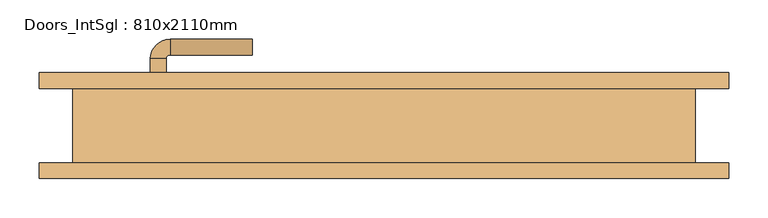
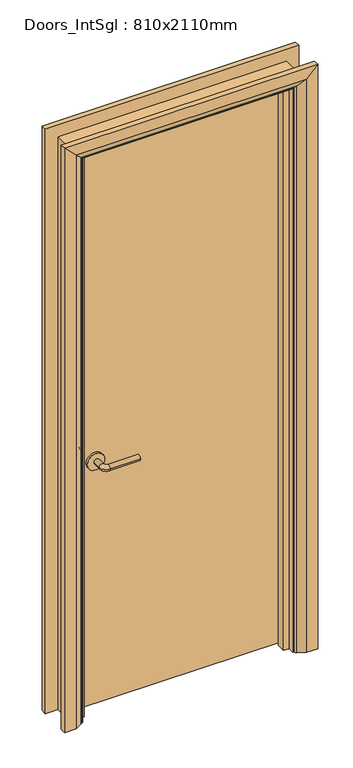
"""IFC4 building model written with IfcOpenShell, lengths in millimetres: door geometry, Doors_IntSgl : 810x2110mm."""

import ifcopenshell
import ifcopenshell.guid

model = None  # the IFC model being written
_history = None  # IfcOwnerHistory: only IFC2X3 demands one
_inside = {}  # id of a spatial element -> (the spatial element, [elements in it])
_under = {}  # id of a project, library or spatial element -> (it, [spatial elements below it])
_declared = {}  # id of a project -> (the project, [libraries it declares])
_typed = {}  # id of a type object -> (the type object, [elements of that type])
_made_of = {}  # id of a material, layer set ... -> (it, [elements and type objects made of it])


def new_model(schema):
    """Start an empty IFC model of exactly this schema.

    Asked for "IFC4X3", IfcOpenShell would pick the latest addendum, in which some entities
    have other attributes; the version numbers below select the first issue.
    IFC2X3 requires an IfcOwnerHistory on every rooted entity: one is made here for all.
    """
    global model, _history
    if schema == "IFC4X3":
        model = ifcopenshell.file(schema_version=(4, 3, 0, 0))
    else:
        model = ifcopenshell.file(schema=schema)
    _inside.clear()
    _under.clear()
    _declared.clear()
    _typed.clear()
    _made_of.clear()
    _history = None
    if model.schema == "IFC2X3":
        org = make("IfcOrganization", Name="unknown")
        user = make(
            "IfcPersonAndOrganization",
            ThePerson=make("IfcPerson", FamilyName="unknown"),
            TheOrganization=org,
        )
        app = make(
            "IfcApplication",
            ApplicationDeveloper=org,
            Version="unknown",
            ApplicationFullName="unknown",
            ApplicationIdentifier="unknown",
        )
        _history = make(
            "IfcOwnerHistory",
            OwningUser=user,
            OwningApplication=app,
            ChangeAction="ADDED",
            CreationDate=0,
        )
    return model


def make(cls, **values):
    """One entity of the class cls with the attributes given. An attribute that is None is left unset."""
    return model.create_entity(
        cls, **{name: value for name, value in values.items() if value is not None}
    )


def rooted(cls, **values):
    """An entity with a GlobalId (a new one), such as an element, a storey or a relation."""
    return make(cls, GlobalId=ifcopenshell.guid.new(), OwnerHistory=_history, **values)


def si_unit(unit_type, name, prefix=None):
    """IfcSIUnit, for example si_unit("LENGTHUNIT", "METRE", prefix="MILLI")."""
    return make("IfcSIUnit", UnitType=unit_type, Prefix=prefix, Name=name)


def assignment(units):
    """IfcUnitAssignment: the units of a project."""
    return None if units is None else make("IfcUnitAssignment", Units=units)


def point(xyz):
    """IfcCartesianPoint."""
    return None if xyz is None else make("IfcCartesianPoint", Coordinates=xyz)


def direction(xyz):
    """IfcDirection."""
    return None if xyz is None else make("IfcDirection", DirectionRatios=xyz)


def frame(location, z_axis=None, x_axis=None):
    """IfcAxis2Placement3D, a coordinate frame: its origin and axes. An axis left out is left unset."""
    return make(
        "IfcAxis2Placement3D",
        Location=point(location),
        Axis=direction(z_axis),
        RefDirection=direction(x_axis),
    )


def frame_2d(location, x_axis=None):
    """IfcAxis2Placement2D, a coordinate frame in the plane: its origin and x axis."""
    return make(
        "IfcAxis2Placement2D", Location=point(location), RefDirection=direction(x_axis)
    )


def origin():
    """The frame at (0, 0, 0) with its axes left unset."""
    return frame((0.0, 0.0, 0.0))


def place(relative_to, where):
    """IfcLocalPlacement: puts the frame where relative to a parent placement (None: the world)."""
    return make(
        "IfcLocalPlacement", PlacementRelTo=relative_to, RelativePlacement=where
    )


def context(
    kind, dimensions, precision=None, world=None, true_north=None, identifier=None
):
    """IfcGeometricRepresentationContext, for example the 3D "Model" context."""
    return make(
        "IfcGeometricRepresentationContext",
        ContextIdentifier=identifier,
        ContextType=kind,
        CoordinateSpaceDimension=dimensions,
        Precision=precision,
        WorldCoordinateSystem=world,
        TrueNorth=true_north,
    )


def project(units=None, contexts=None):
    """IfcProject with its units and contexts."""
    return rooted(
        "IfcProject",
        Name="project",
        RepresentationContexts=contexts,
        UnitsInContext=assignment(units),
    )


def spatial(cls, under=None, at=None, **own):
    """A site, building, storey or space (cls), placed at a placement, below another one or the project."""
    s = rooted(cls, ObjectPlacement=at, **own)
    if under is not None:
        _under.setdefault(under.id(), (under, []))[1].append(s)
    return s


def polyline(points):
    """IfcPolyline through the points."""
    return make("IfcPolyline", Points=[point(p) for p in points])


def circle_curve(where, radius):
    """IfcCircle in the frame where."""
    return make("IfcCircle", Position=where, Radius=radius)


def ellipse_curve(where, semi_axis1, semi_axis2):
    """IfcEllipse in the frame where."""
    return make(
        "IfcEllipse", Position=where, SemiAxis1=semi_axis1, SemiAxis2=semi_axis2
    )


def trimmed(basis, trim1, trim2, sense, master):
    """IfcTrimmedCurve: the piece of a basis curve between two trims."""
    return make(
        "IfcTrimmedCurve",
        BasisCurve=basis,
        Trim1=trim1,
        Trim2=trim2,
        SenseAgreement=sense,
        MasterRepresentation=master,
    )


def segment(curve, same_sense, transition):
    """IfcCompositeCurveSegment."""
    return make(
        "IfcCompositeCurveSegment",
        Transition=transition,
        SameSense=same_sense,
        ParentCurve=curve,
    )


def composite_curve(segments, self_intersect=None):
    """IfcCompositeCurve: segments joined end to end."""
    return make("IfcCompositeCurve", Segments=segments, SelfIntersect=self_intersect)


def outline(outer, holes=None, kind="AREA"):
    """IfcArbitraryClosedProfileDef: a profile drawn as a closed curve; with holes, ...WithVoids."""
    if holes is None:
        return make("IfcArbitraryClosedProfileDef", ProfileType=kind, OuterCurve=outer)
    return make(
        "IfcArbitraryProfileDefWithVoids",
        ProfileType=kind,
        OuterCurve=outer,
        InnerCurves=holes,
    )


def extrude(swept, where, along, depth):
    """IfcExtrudedAreaSolid: the profile swept, set in the frame where, extruded along a direction by depth."""
    return make(
        "IfcExtrudedAreaSolid",
        SweptArea=swept,
        Position=where,
        ExtrudedDirection=direction(along),
        Depth=depth,
    )


def faces_of(points, faces, orient=None, outer=None):
    """IfcFace entities. A face is a list of loops; a loop is a list of indices into points, from 0.

    orient and outer hold one flag for each loop. By default every Orientation is true, the
    first loop of a face is its IfcFaceOuterBound and the others are IfcFaceBound.
    """
    made = []
    for i, loops in enumerate(faces):
        bounds = []
        for j, loop in enumerate(loops):
            is_outer = j == 0 if outer is None else outer[i][j]
            bounds.append(
                make(
                    "IfcFaceOuterBound" if is_outer else "IfcFaceBound",
                    Bound=make("IfcPolyLoop", Polygon=[points[k] for k in loop]),
                    Orientation=True if orient is None else orient[i][j],
                )
            )
        made.append(make("IfcFace", Bounds=bounds))
    return made


def faceted_brep(points, faces, orient=None, outer=None, voids=None):
    """IfcFacetedBrep: a solid bounded by flat faces; with voids (closed shells), ...WithVoids."""
    shared = [point(p) for p in points]
    hull = make("IfcClosedShell", CfsFaces=faces_of(shared, faces, orient, outer))
    if voids is None:
        return make("IfcFacetedBrep", Outer=hull)
    return make(
        "IfcFacetedBrepWithVoids",
        Outer=hull,
        Voids=[
            make(cls, CfsFaces=faces_of(shared, fs, o, b)) for cls, fs, o, b in voids
        ],
    )


def shape(context_of_items, identifier, shape_type, items):
    """IfcShapeRepresentation: the items that make up one representation, for example the "Body"."""
    return make(
        "IfcShapeRepresentation",
        ContextOfItems=context_of_items,
        RepresentationIdentifier=identifier,
        RepresentationType=shape_type,
        Items=items,
    )


def source(mapping_origin, context_of_items, identifier, shape_type, items):
    """IfcRepresentationMap: a shape defined once, which mapped items show again and again."""
    return make(
        "IfcRepresentationMap",
        MappingOrigin=mapping_origin,
        MappedRepresentation=shape(context_of_items, identifier, shape_type, items),
    )


def transform(
    local_origin,
    x_axis=None,
    y_axis=None,
    z_axis=None,
    scale=None,
    scale2=None,
    scale3=None,
    uniform=True,
):
    """IfcCartesianTransformationOperator3D, or its non-uniform kind. x_axis, y_axis, z_axis: its Axis1, 2, 3."""
    if uniform:
        return make(
            "IfcCartesianTransformationOperator3D",
            Axis1=direction(x_axis),
            Axis2=direction(y_axis),
            LocalOrigin=point(local_origin),
            Scale=scale,
            Axis3=direction(z_axis),
        )
    return make(
        "IfcCartesianTransformationOperator3DnonUniform",
        Axis1=direction(x_axis),
        Axis2=direction(y_axis),
        LocalOrigin=point(local_origin),
        Scale=scale,
        Axis3=direction(z_axis),
        Scale2=scale2,
        Scale3=scale3,
    )


def mapped(mapping_source, mapping_target):
    """IfcMappedItem: shows the shape of a source again, moved by a transform."""
    return make(
        "IfcMappedItem", MappingSource=mapping_source, MappingTarget=mapping_target
    )


def made_of(thing, what):
    """Note that an element or type object is made of a material, layer set ...; save() writes the relation."""
    if what is not None:
        _made_of.setdefault(what.id(), (what, []))[1].append(thing)
    return thing


def element(
    cls,
    number,
    at=None,
    inside=None,
    cuts=None,
    type_object=None,
    material=None,
    context=None,
    identifier="Body",
    shape_type=None,
    held_by="IfcProductDefinitionShape",
    body=None,
    shapes=None,
    **own,
):
    """One element of the class cls, such as IfcWall. Its Tag is "e" and its number.

    at: its placement. inside: the storey or other place that contains it. cuts: it is an
    opening in that element (IfcRelVoidsElement). A single representation is given by context,
    identifier, shape_type and body (its items); several are given by shapes. held_by: the class
    of the entity that holds the representations. save() writes the other relations.
    """
    e = rooted(cls, Tag="e%d" % number, ObjectPlacement=at, **own)
    if body is not None:
        shapes = [shape(context, identifier, shape_type, body)]
    if shapes is not None:
        e.Representation = make(held_by, Representations=shapes)
    if inside is not None:
        _inside.setdefault(inside.id(), (inside, []))[1].append(e)
    if cuts is not None:
        rooted(
            "IfcRelVoidsElement", RelatingBuildingElement=cuts, RelatedOpeningElement=e
        )
    if type_object is not None:
        _typed.setdefault(type_object.id(), (type_object, []))[1].append(e)
    return made_of(e, material)


def aggregate(whole, parts):
    """IfcRelAggregates: a whole, such as a stair, and the parts it consists of."""
    return rooted("IfcRelAggregates", RelatingObject=whole, RelatedObjects=parts)


def save(model, path):
    """Write the relations noted so far, then the file.

    IfcRelAggregates (storeys below a building ...), IfcRelContainedInSpatialStructure (elements
    in a storey), IfcRelDefinesByType, IfcRelAssociatesMaterial and IfcRelDeclares: one each for
    every whole, place, type object, material and project.
    """
    for whole, parts in _under.values():
        aggregate(whole, parts)
    for where, things in _inside.values():
        rooted(
            "IfcRelContainedInSpatialStructure",
            RelatedElements=things,
            RelatingStructure=where,
        )
    for kind, things in _typed.values():
        rooted("IfcRelDefinesByType", RelatedObjects=things, RelatingType=kind)
    for what, things in _made_of.values():
        rooted("IfcRelAssociatesMaterial", RelatedObjects=things, RelatingMaterial=what)
    for by, libraries in _declared.values():
        rooted("IfcRelDeclares", RelatingContext=by, RelatedDefinitions=libraries)
    model.write(path)


def plane_surface(at):
    """IfcPlane: the flat surface through the origin of the frame at, square to its z axis."""
    return make("IfcPlane", Position=at)


def cylinder_surface(at, radius):
    """IfcCylindricalSurface: all points at the distance radius from the z axis of the frame at."""
    return make("IfcCylindricalSurface", Position=at, Radius=radius)


def revolved_surface(curve, axis_point, axis_direction):
    """IfcSurfaceOfRevolution: the curve turned about the line through axis_point along axis_direction."""
    return make(
        "IfcSurfaceOfRevolution",
        SweptCurve=make("IfcArbitraryOpenProfileDef", ProfileType="CURVE", Curve=curve),
        AxisPosition=make("IfcAxis1Placement", Location=point(axis_point), Axis=direction(axis_direction)),
    )


def advanced_brep(points, edges, surfaces, faces):
    """IfcAdvancedBrep: a solid bounded by faces that lie on surfaces and meet in shared edges.

    An edge is (start, end): straight between two places in points (the first is 0);
    or (start, end, curve); or (start, end, curve, False) where it runs against its curve.
    A face is (place in surfaces, loops), or (place, loops, False) where it looks against
    its surface's normal. A loop lists edges by number (the first is 1), with a minus sign
    where the edge is run from its end to its start. The first loop is the outer one.
    """
    corners = [point(p) for p in points]
    vertices = [make("IfcVertexPoint", VertexGeometry=c) for c in corners]
    made = []
    for start, end, *more in edges:
        made.append(
            make(
                "IfcEdgeCurve",
                EdgeStart=vertices[start],
                EdgeEnd=vertices[end],
                EdgeGeometry=more[0] if more else make("IfcPolyline", Points=[corners[start], corners[end]]),
                SameSense=more[1] if len(more) > 1 else True,
            )
        )
    hull = []
    for where, loops, *sense in faces:
        bounds = []
        for j, loop in enumerate(loops):
            ring = [make("IfcOrientedEdge", EdgeElement=made[abs(k) - 1], Orientation=k > 0) for k in loop]
            bounds.append(
                make(
                    "IfcFaceOuterBound" if j == 0 else "IfcFaceBound",
                    Bound=make("IfcEdgeLoop", EdgeList=ring),
                    Orientation=True,
                )
            )
        hull.append(make("IfcAdvancedFace", Bounds=bounds, FaceSurface=surfaces[where], SameSense=sense[0] if sense else True))
    return make("IfcAdvancedBrep", Outer=make("IfcClosedShell", CfsFaces=hull))


def doors_intsgl_810x2110mm_acea5367(model_context):
    return source(origin(), model_context, "Body", "SolidModel", [
        advanced_brep(
        [(-298.0, 1.5, 900.0), (-278.0, 1.5, 900.0), (-278.0, -28.5, 900.0), (-298.0, -28.5, 900.0), (-273.0, -33.5, 900.0), (-273.0, -53.5, 900.0), (-168.0, -53.5, 900.0), (-168.0, -33.5, 900.0)],
        [
            (0, 1, circle_curve(frame((-288.0, 1.5, 900.0), z_axis=(0.0, 1.0, 0.0), x_axis=(1.0, 0.0, 0.0)), 10.0)),
            (1, 0, circle_curve(frame((-288.0, 1.5, 900.0), z_axis=(0.0, 1.0, 0.0), x_axis=(1.0, 0.0, 0.0)), 10.0)),
            (1, 2),
            (2, 3, circle_curve(frame((-288.0, -28.5, 900.0), z_axis=(0.0, 1.0, 0.0), x_axis=(1.0, 0.0, 0.0)), 10.0)),
            (3, 0),
            (3, 2, circle_curve(frame((-288.0, -28.5, 900.0), z_axis=(0.0, 1.0, 0.0), x_axis=(1.0, 0.0, 0.0)), 10.0)),
            (4, 5, circle_curve(frame((-273.0, -43.5, 900.0), z_axis=(-1.0, 0.0, 0.0), x_axis=(0.0, 1.0, 0.0)), 10.0)),
            (5, 3, circle_curve(frame((-273.0, -28.5, 900.0), z_axis=(0.0, 0.0, -1.0), x_axis=(-1.0, 0.0, 0.0)), 25.0)),
            (2, 4, circle_curve(frame((-273.0, -28.5, 900.0), z_axis=(0.0, 0.0, 1.0), x_axis=(-1.0, 0.0, 0.0)), 5.0)),
            (5, 4, circle_curve(frame((-273.0, -43.5, 900.0), z_axis=(-1.0, 0.0, 0.0), x_axis=(0.0, 1.0, 0.0)), 10.0)),
            (6, 7, circle_curve(frame((-168.0, -43.5, 900.0), z_axis=(1.0, 0.0, 0.0), x_axis=(0.0, 1.0, 0.0)), 10.0)),
            (7, 6, circle_curve(frame((-168.0, -43.5, 900.0), z_axis=(1.0, 0.0, 0.0), x_axis=(0.0, 1.0, 0.0)), 10.0)),
            (4, 7),
            (6, 5),
        ],
        [
            plane_surface(frame((-288.0, 1.5, 900.0), z_axis=(0.0, 1.0, 0.0), x_axis=(0.0, 0.0, 1.0))),
            cylinder_surface(frame((-288.0, 1.5, 900.0), z_axis=(0.0, 1.0, 0.0), x_axis=(1.0, 0.0, 0.0)), 10.0),
            revolved_surface(trimmed(ellipse_curve(frame((-288.0, -28.5, 900.0), z_axis=(0.0, -1.0, 0.0), x_axis=(1.0, 0.0, 0.0)), 10.0, 10.0), [point((-298.0, -28.5, 900.0))], [point((-278.0, -28.5, 900.0))], True, "CARTESIAN"), (-273.0, -28.5, 900.0), (0.0, 0.0, -1.0)),
            revolved_surface(trimmed(ellipse_curve(frame((-288.0, -28.5, 900.0), z_axis=(0.0, -1.0, 0.0), x_axis=(1.0, 0.0, 0.0)), 10.0, 10.0), [point((-278.0, -28.5, 900.0))], [point((-298.0, -28.5, 900.0))], True, "CARTESIAN"), (-273.0, -28.5, 900.0), (0.0, 0.0, -1.0)),
            plane_surface(frame((-168.0, -43.5, 900.0), z_axis=(1.0, 0.0, 0.0), x_axis=(0.0, 0.0, 1.0))),
            cylinder_surface(frame((-273.0, -43.5, 900.0), z_axis=(-1.0, 0.0, 0.0), x_axis=(0.0, 1.0, 0.0)), 10.0),
        ],
        [
            (0, [[1, 2]]),
            (1, [[3, 4, 5, -2]]),
            (1, [[-5, 6, -3, -1]]),
            (2, [[7, 8, -4, 9]]),
            (3, [[10, -9, -6, -8]]),
            (4, [[11, 12]]),
            (5, [[13, -11, 14, -7]]),
            (5, [[-14, -12, -13, -10]]),
        ],
    ),
        extrude(outline(composite_curve([segment(trimmed(circle_curve(frame_2d((900.0, -290.5)), 30.0), [point((900.0, -320.5))], [point((900.0, -260.5))], False, "CARTESIAN"), True, "CONTINUOUS"), segment(trimmed(circle_curve(frame_2d((900.0, -290.5)), 30.0), [point((900.0, -260.5))], [point((900.0, -320.5))], False, "CARTESIAN"), True, "CONTINUOUS")], self_intersect=False)), frame((0.0, 1.5, 0.0), z_axis=(0.0, 1.0, 0.0), x_axis=(0.0, 0.0, 1.0)), (0.0, 0.0, 1.0), 8.0),
        advanced_brep(
        [(-298.0, 55.5, 900.0), (-278.0, 55.5, 900.0), (-298.0, 85.5, 900.0), (-278.0, 85.5, 900.0), (-273.0, 90.5, 900.0), (-273.0, 110.5, 900.0), (-168.0, 110.5, 900.0), (-168.0, 90.5, 900.0)],
        [
            (0, 1, circle_curve(frame((-288.0, 55.5, 900.0), z_axis=(0.0, -1.0, 0.0), x_axis=(1.0, 0.0, 0.0)), 10.0)),
            (1, 0, circle_curve(frame((-288.0, 55.5, 900.0), z_axis=(0.0, -1.0, 0.0), x_axis=(1.0, 0.0, 0.0)), 10.0)),
            (0, 2),
            (2, 3, circle_curve(frame((-288.0, 85.5, 900.0), z_axis=(0.0, -1.0, 0.0), x_axis=(1.0, 0.0, 0.0)), 10.0)),
            (3, 1),
            (3, 2, circle_curve(frame((-288.0, 85.5, 900.0), z_axis=(0.0, -1.0, 0.0), x_axis=(1.0, 0.0, 0.0)), 10.0)),
            (4, 3, circle_curve(frame((-273.0, 85.5, 900.0), z_axis=(0.0, 0.0, 1.0), x_axis=(-1.0, 0.0, 0.0)), 5.0)),
            (2, 5, circle_curve(frame((-273.0, 85.5, 900.0), z_axis=(0.0, 0.0, -1.0), x_axis=(-1.0, 0.0, 0.0)), 25.0)),
            (5, 4, circle_curve(frame((-273.0, 100.5, 900.0), z_axis=(-1.0, 0.0, 0.0), x_axis=(0.0, -1.0, 0.0)), 10.0)),
            (4, 5, circle_curve(frame((-273.0, 100.5, 900.0), z_axis=(-1.0, 0.0, 0.0), x_axis=(0.0, -1.0, 0.0)), 10.0)),
            (6, 7, circle_curve(frame((-168.0, 100.5, 900.0), z_axis=(1.0, 0.0, 0.0), x_axis=(0.0, -1.0, 0.0)), 10.0)),
            (7, 6, circle_curve(frame((-168.0, 100.5, 900.0), z_axis=(1.0, 0.0, 0.0), x_axis=(0.0, -1.0, 0.0)), 10.0)),
            (5, 6),
            (7, 4),
        ],
        [
            plane_surface(frame((-288.0, 55.5, 900.0), z_axis=(0.0, -1.0, 0.0), x_axis=(0.0, 0.0, 1.0))),
            cylinder_surface(frame((-288.0, 55.5, 900.0), z_axis=(0.0, -1.0, 0.0), x_axis=(1.0, 0.0, 0.0)), 10.0),
            revolved_surface(trimmed(ellipse_curve(frame((-288.0, 85.5, 900.0), z_axis=(0.0, -1.0, 0.0), x_axis=(1.0, 0.0, 0.0)), 10.0, 10.0), [point((-298.0, 85.5, 900.0))], [point((-278.0, 85.5, 900.0))], True, "CARTESIAN"), (-273.0, 85.5, 900.0), (0.0, 0.0, -1.0)),
            revolved_surface(trimmed(ellipse_curve(frame((-288.0, 85.5, 900.0), z_axis=(0.0, -1.0, 0.0), x_axis=(1.0, 0.0, 0.0)), 10.0, 10.0), [point((-278.0, 85.5, 900.0))], [point((-298.0, 85.5, 900.0))], True, "CARTESIAN"), (-273.0, 85.5, 900.0), (0.0, 0.0, -1.0)),
            plane_surface(frame((-168.0, 100.5, 900.0), z_axis=(1.0, 0.0, 0.0), x_axis=(0.0, 0.0, 1.0))),
            cylinder_surface(frame((-273.0, 100.5, 900.0), z_axis=(-1.0, 0.0, 0.0), x_axis=(0.0, -1.0, 0.0)), 10.0),
        ],
        [
            (0, [[1, 2]]),
            (1, [[-1, 3, 4, 5]]),
            (1, [[-2, -5, 6, -3]]),
            (2, [[7, -4, 8, 9]]),
            (3, [[-8, -6, -7, 10]]),
            (4, [[11, 12]]),
            (5, [[-9, 13, -12, 14]]),
            (5, [[-10, -14, -11, -13]]),
        ],
    ),
        extrude(outline(composite_curve([segment(trimmed(circle_curve(frame_2d((900.0, -290.5)), 30.0), [point((900.0, -320.5))], [point((900.0, -260.5))], False, "CARTESIAN"), True, "CONTINUOUS"), segment(trimmed(circle_curve(frame_2d((900.0, -290.5)), 30.0), [point((900.0, -260.5))], [point((900.0, -320.5))], False, "CARTESIAN"), True, "CONTINUOUS")], self_intersect=False)), frame((0.0, 47.5, 0.0), z_axis=(0.0, 1.0, 0.0), x_axis=(0.0, 0.0, 1.0)), (0.0, 0.0, 1.0), 8.0),
        extrude(outline(polyline([(363.0, 9.5), (-363.0, 9.5), (-363.0, 47.5), (363.0, 47.5), (363.0, 9.5)])), frame((0.0, 0.0, 8.0), z_axis=(0.0, 0.0, 1.0), x_axis=(1.0, 0.0, 0.0)), (0.0, 0.0, 1.0), 2060.0),
        advanced_brep(
        [(440.0, 67.5, 0.0), (440.0, 47.5, 0.0), (370.0, 47.5, 0.0), (374.0, 53.5, 0.0), (400.0, 67.5, 0.0), (440.0, 67.5, 2145.0), (440.0, 47.5, 2145.0), (-440.0, 47.5, 2145.0), (-440.0, 47.5, 0.0), (-370.0, 47.5, 0.0), (-370.0, 47.5, 2075.0), (370.0, 47.5, 2075.0), (374.0, 53.5, 2079.0), (400.0, 67.5, 2105.0), (-400.0, 67.5, 2105.0), (-400.0, 67.5, 0.0), (-440.0, 67.5, 0.0), (-440.0, 67.5, 2145.0), (-374.0, 53.5, 2079.0), (-374.0, 53.5, 0.0)],
        [
            (0, 1),
            (1, 2),
            (2, 3, circle_curve(frame((378.0, 46.5, 0.0), z_axis=(0.0, 0.0, -1.0), x_axis=(1.0, 0.0, 0.0)), 8.0622577)),
            (3, 4),
            (4, 0),
            (0, 5),
            (5, 6),
            (6, 1),
            (6, 7),
            (7, 8),
            (8, 9),
            (9, 10),
            (10, 11),
            (11, 2),
            (11, 12, ellipse_curve(frame((378.0, 46.5, 2083.0), z_axis=(0.7071067811865475, 0.0, -0.7071067811865475), x_axis=(-0.7071067811865474, 0.0, -0.7071067811865476)), 11.4017543, 8.0622577)),
            (12, 3),
            (12, 13),
            (13, 4),
            (13, 14),
            (14, 15),
            (15, 16),
            (16, 17),
            (17, 5),
            (17, 7),
            (10, 18, ellipse_curve(frame((-378.0, 46.5, 2083.0), z_axis=(0.7071067811865475, 0.0, 0.7071067811865475), x_axis=(0.7071067811865476, 0.0, -0.7071067811865474)), 11.4017543, 8.0622577)),
            (18, 12),
            (18, 14),
            (15, 19),
            (19, 9, circle_curve(frame((-378.0, 46.5, 0.0), z_axis=(0.0, 0.0, -1.0), x_axis=(-1.0, 0.0, 0.0)), 8.0622577)),
            (8, 16),
            (19, 18),
        ],
        [
            plane_surface(frame((370.0, 47.5, 0.0), z_axis=(0.0, 0.0, -1.0), x_axis=(0.0, -1.0, 0.0))),
            plane_surface(frame((440.0, 67.5, 0.0), z_axis=(1.0, 0.0, 0.0), x_axis=(0.0, 0.0, 1.0))),
            plane_surface(frame((440.0, 47.5, 0.0), z_axis=(0.0, -1.0, 0.0), x_axis=(0.0, 0.0, 1.0))),
            cylinder_surface(frame((378.0, 46.5, 0.0), z_axis=(0.0, 0.0, -1.0), x_axis=(1.0, 0.0, 0.0)), 8.0622577),
            plane_surface(frame((374.0, 53.5, 0.0), z_axis=(-0.4740998230350126, 0.880471099922178, 0.0), x_axis=(0.0, 0.0, 1.0))),
            plane_surface(frame((400.0, 67.5, 0.0), z_axis=(0.0, 1.0, 0.0), x_axis=(0.0, 0.0, 1.0))),
            plane_surface(frame((440.0, 67.5, 2145.0), z_axis=(0.0, 0.0, 1.0), x_axis=(-1.0, 0.0, 0.0))),
            cylinder_surface(frame((370.0, 46.5, 2083.0), z_axis=(1.0, 0.0, 0.0), x_axis=(0.0, 0.0, 1.0)), 8.0622577),
            plane_surface(frame((374.0, 53.5, 2079.0), z_axis=(0.0, 0.8804710999221764, -0.4740998230350154), x_axis=(-1.0, 0.0, 0.0))),
            plane_surface(frame((-370.0, 47.5, 0.0), z_axis=(0.0, 0.0, -1.0), x_axis=(0.0, -1.0, 0.0))),
            plane_surface(frame((-440.0, 67.5, 2145.0), z_axis=(-1.0, 0.0, 0.0), x_axis=(0.0, 0.0, -1.0))),
            cylinder_surface(frame((-378.0, 46.5, 2075.0), z_axis=(0.0, 0.0, 1.0), x_axis=(-1.0, 0.0, 0.0)), 8.0622577),
            plane_surface(frame((-374.0, 53.5, 2079.0), z_axis=(0.47409982303501824, 0.8804710999221749, 0.0), x_axis=(0.0, 0.0, -1.0))),
        ],
        [
            (0, [[1, 2, 3, 4, 5]]),
            (1, [[-1, 6, 7, 8]]),
            (2, [[-2, -8, 9, 10, 11, 12, 13, 14]]),
            (3, [[-3, -14, 15, 16]]),
            (4, [[-4, -16, 17, 18]]),
            (5, [[-5, -18, 19, 20, 21, 22, 23, -6]]),
            (6, [[-7, -23, 24, -9]]),
            (7, [[-15, -13, 25, 26]]),
            (8, [[-17, -26, 27, -19]]),
            (9, [[-21, 28, 29, -11, 30]]),
            (10, [[-24, -22, -30, -10]]),
            (11, [[-25, -12, -29, 31]]),
            (12, [[-27, -31, -28, -20]]),
        ],
    ),
        extrude(outline(polyline([(0.0, -365.0), (0.0, -346.0), (2051.0, -346.0), (2051.0, 346.0), (0.0, 346.0), (0.0, 365.0), (2070.0, 365.0), (2070.0, -365.0), (0.0, -365.0)])), frame((0.0, -24.5, 0.0), z_axis=(0.0, 1.0, 0.0), x_axis=(0.0, 0.0, 1.0)), (0.0, 0.0, 1.0), 32.0),
        advanced_brep(
        [(-440.0, -67.5, 0.0), (-440.0, -47.5, 0.0), (-370.0, -47.5, 0.0), (-374.0, -53.5, 0.0), (-400.0, -67.5, 0.0), (-440.0, -67.5, 2145.0), (-440.0, -47.5, 2145.0), (-370.0, -47.5, 2075.0), (-374.0, -53.5, 2079.0), (-400.0, -67.5, 2105.0), (440.0, -67.5, 2145.0), (440.0, -47.5, 2145.0), (370.0, -47.5, 2075.0), (374.0, -53.5, 2079.0), (400.0, -67.5, 2105.0), (440.0, -67.5, 0.0), (400.0, -67.5, 0.0), (374.0, -53.5, 0.0), (370.0, -47.5, 0.0), (440.0, -47.5, 0.0)],
        [
            (0, 1),
            (1, 2),
            (2, 3, circle_curve(frame((-378.0, -46.5, 0.0), z_axis=(0.0, 0.0, -1.0), x_axis=(-1.0, 0.0, 0.0)), 8.0622577)),
            (3, 4),
            (4, 0),
            (0, 5),
            (5, 6),
            (6, 1),
            (6, 7),
            (7, 2),
            (7, 8, ellipse_curve(frame((-378.0, -46.5, 2083.0), z_axis=(-0.7071067811865475, 0.0, -0.7071067811865475), x_axis=(0.7071067811865474, 0.0, -0.7071067811865476)), 11.4017543, 8.0622577)),
            (8, 3),
            (8, 9),
            (9, 4),
            (9, 5),
            (5, 10),
            (10, 11),
            (11, 6),
            (11, 12),
            (12, 7),
            (12, 13, ellipse_curve(frame((378.0, -46.5, 2083.0), z_axis=(-0.7071067811865475, 0.0, 0.7071067811865475), x_axis=(-0.7071067811865476, 0.0, -0.7071067811865474)), 11.4017543, 8.0622577)),
            (13, 8),
            (13, 14),
            (14, 9),
            (14, 10),
            (15, 16),
            (16, 17),
            (17, 18, circle_curve(frame((378.0, -46.5, 0.0), z_axis=(0.0, 0.0, -1.0), x_axis=(1.0, 0.0, 0.0)), 8.0622577)),
            (18, 19),
            (19, 15),
            (10, 15),
            (19, 11),
            (18, 12),
            (17, 13),
            (16, 14),
        ],
        [
            plane_surface(frame((-370.0, -120.3010989, 0.0), z_axis=(0.0, 0.0, -1.0), x_axis=(1.0, 0.0, 0.0))),
            plane_surface(frame((-440.0, -67.5, 0.0), z_axis=(-1.0, 0.0, 0.0), x_axis=(0.0, 0.0, 1.0))),
            plane_surface(frame((-440.0, -47.5, 0.0), z_axis=(0.0, 1.0, 0.0), x_axis=(0.0, 0.0, 1.0))),
            cylinder_surface(frame((-378.0, -46.5, 0.0), z_axis=(0.0, 0.0, -1.0), x_axis=(-1.0, 0.0, 0.0)), 8.0622577),
            plane_surface(frame((-374.0, -53.5, 0.0), z_axis=(0.4740998230350183, -0.8804710999221749, 0.0), x_axis=(0.0, 0.0, 1.0))),
            plane_surface(frame((-400.0, -67.5, 0.0), z_axis=(0.0, -1.0, 0.0), x_axis=(0.0, 0.0, 1.0))),
            plane_surface(frame((-440.0, -67.5, 2145.0), z_axis=(0.0, 0.0, 1.0), x_axis=(1.0, 0.0, 0.0))),
            plane_surface(frame((-440.0, -47.5, 2145.0), z_axis=(0.0, 1.0, 0.0), x_axis=(1.0, 0.0, 0.0))),
            cylinder_surface(frame((-370.0, -46.5, 2083.0), z_axis=(-1.0, 0.0, 0.0), x_axis=(0.0, 0.0, 1.0)), 8.0622577),
            plane_surface(frame((-374.0, -53.5, 2079.0), z_axis=(0.0, -0.8804710999221749, -0.4740998230350183), x_axis=(1.0, 0.0, 0.0))),
            plane_surface(frame((-400.0, -67.5, 2105.0), z_axis=(0.0, -1.0, 0.0), x_axis=(1.0, 0.0, 0.0))),
            plane_surface(frame((370.0, -120.3010989, 0.0), z_axis=(0.0, 0.0, -1.0), x_axis=(-1.0, 0.0, 0.0))),
            plane_surface(frame((440.0, -67.5, 2145.0), z_axis=(1.0, 0.0, 0.0), x_axis=(0.0, 0.0, -1.0))),
            plane_surface(frame((440.0, -47.5, 2145.0), z_axis=(0.0, 1.0, 0.0), x_axis=(0.0, 0.0, -1.0))),
            cylinder_surface(frame((378.0, -46.5, 2075.0), z_axis=(0.0, 0.0, 1.0), x_axis=(1.0, 0.0, 0.0)), 8.0622577),
            plane_surface(frame((374.0, -53.5, 2079.0), z_axis=(-0.4740998230350183, -0.8804710999221749, 0.0), x_axis=(0.0, 0.0, -1.0))),
            plane_surface(frame((400.0, -67.5, 2105.0), z_axis=(0.0, -1.0, 0.0), x_axis=(0.0, 0.0, -1.0))),
        ],
        [
            (0, [[1, 2, 3, 4, 5]]),
            (1, [[-1, 6, 7, 8]]),
            (2, [[-2, -8, 9, 10]]),
            (3, [[-3, -10, 11, 12]]),
            (4, [[-4, -12, 13, 14]]),
            (5, [[-5, -14, 15, -6]]),
            (6, [[-7, 16, 17, 18]]),
            (7, [[-9, -18, 19, 20]]),
            (8, [[-11, -20, 21, 22]]),
            (9, [[-13, -22, 23, 24]]),
            (10, [[-15, -24, 25, -16]]),
            (11, [[26, 27, 28, 29, 30]]),
            (12, [[-17, 31, -30, 32]]),
            (13, [[-19, -32, -29, 33]]),
            (14, [[-21, -33, -28, 34]]),
            (15, [[-23, -34, -27, 35]]),
            (16, [[-25, -35, -26, -31]]),
        ],
    ),
        faceted_brep([(-365.0, 47.5, 0.0), (-365.0, -47.5, 0.0), (-397.0, -47.5, 0.0), (-397.0, 47.5, 0.0), (-365.0, 47.5, 2070.0), (-365.0, -47.5, 2070.0), (-397.0, -47.5, 2102.0), (-397.0, 47.5, 2102.0), (365.0, 47.5, 2070.0), (365.0, -47.5, 2070.0), (397.0, -47.5, 2102.0), (397.0, 47.5, 2102.0), (365.0, 47.5, 0.0), (397.0, 47.5, 0.0), (397.0, -47.5, 0.0), (365.0, -47.5, 0.0)], [[[0, 1, 2, 3]], [[1, 0, 4, 5]], [[2, 1, 5, 6]], [[3, 2, 6, 7]], [[0, 3, 7, 4]], [[5, 4, 8, 9]], [[6, 5, 9, 10]], [[7, 6, 10, 11]], [[4, 7, 11, 8]], [[12, 13, 14, 15]], [[9, 8, 12, 15]], [[10, 9, 15, 14]], [[11, 10, 14, 13]], [[8, 11, 13, 12]]]),
    ])


if __name__ == "__main__":
    model = new_model("IFC4")
    model_context = context("Model", 3, world=origin())
    ifc_project = project(units=[si_unit("LENGTHUNIT", "METRE", prefix="MILLI")], contexts=[model_context])
    site = spatial("IfcSite", under=ifc_project)
    building = spatial("IfcBuilding", under=site)
    placement = place(None, origin())
    doors_intsgl_810x2110mm_shape = doors_intsgl_810x2110mm_acea5367(model_context)
    element("IfcDoor", 1, ObjectType="Doors_IntSgl : 810x2110mm", at=placement, inside=building, context=model_context, shape_type="MappedRepresentation", body=[
        mapped(doors_intsgl_810x2110mm_shape, transform((0.0, 0.0, 0.0), x_axis=(1.0, 0.0, 0.0), y_axis=(0.0, 1.0, 0.0), z_axis=(0.0, 0.0, 1.0))),
    ])
    save(model, "model.ifc")

# Revit data of these elements
# Type "Doors_IntSgl : 810x2110mm"
#   Construction Type Id = "MDOOR"
#   Type Mark = "42"
#   Type Comments = "Internal Single"
#   Operation = "SingleSwingRight"
#   Manufacturer = "Revit"
#   Keynote = "L20"
#   Description = "Internal Single Door"
#   Analytic Construction = "Metal"
#   UnderCut = 8 mm
#   Tolerance = 2 mm
#   Thickness = 38 mm
#   Thermal Resistance (R) = 0.270117 (m²·K)/W
#   Structural Tolerance = 8 mm
#   StopDepth = 32 mm
#   Stop Thickness = 19 mm
#   Rough Width = 810 mm
#   Rough Height = 2110 mm
#   Height to Top Lock Rail = 1000 mm
#   Heat Transfer Coefficient (U) = 3.7021 W/(m²·K)
#   Handle Z Distance = 900 mm
#   Handle X Distance = 75 mm
#   Frame Thickness = 32 mm
#   Door Panel Width = 726 mm
#   Door Panel Thickness = 38 mm
#   Door Panel Offset = 0 mm
#   Height = 2110 mm
#   Width = 810 mm
#   Door Panel Height = 2060 mm
#   Architrave Setback = 5 mm
#   Vis - Ironmongery = yes
#   Material Ironmongery = Door - Handle
#   Material Frame = Door - Frame/Mullion (1)
#   Material Door = Door - Panel
#   Material Architrave = Door - Architrave
#   Visual Light Transmittance = 0
#   Solar Heat Gain Coefficient = 0
#   Function = (empty or 0)
#   Wall Closure = (empty or 0)
# Element 1 (IfcDoor, "Doors_IntSgl : 810x2110mm")
#   Materials on its faces: "Door - Architrave", "Door - Handle", "Door - Frame/Mullion (1)", "Door - Panel"
# Materials
#   "Door - Handle": class "Miscellaneous", colour RGB 0 0 0, transparency 0, Keynote = "P21", Cost = 0
#   "Door - Frame/Mullion (1)": class "Wood", colour RGB 212 179 113, transparency 0, Keynote = "L20", Cost = 0
#   "Door - Panel": class "Wood", colour RGB 210 159 95, transparency 0, Keynote = "L20", Cost = 0
#   "Door - Architrave": class "Wood", colour RGB 154 90 5, transparency 0, Keynote = "P20", Cost = 0
